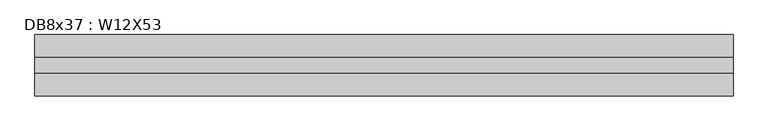
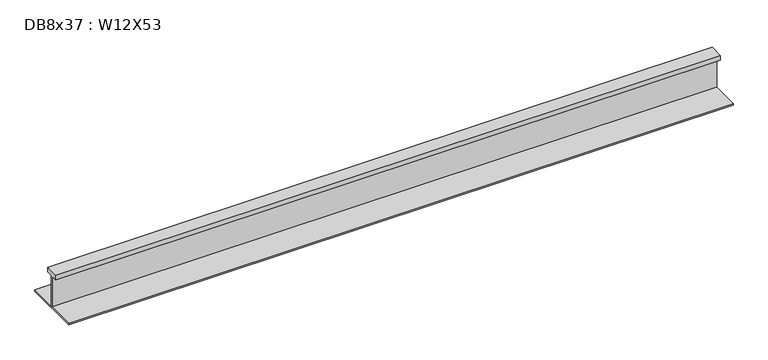
"""IFC4 building model written with IfcOpenShell, lengths in millimetres: beam geometry, DB8x37 : W12X53."""

from ifc_helpers import new_model, si_unit, frame, origin, place, context, project, spatial, polyline, outline, extrude, source, transform, mapped, element, save


def db8x37_w12x53_a618b606(model_context):
    return source(origin(), model_context, "Body", "SweptSolid", [
        extrude(outline(polyline([(38.1, 145.415), (38.1, 120.015), (2.921, 120.015), (2.921, -48.4505), (152.4, -48.4505), (152.4, -58.1025), (-152.4, -58.1025), (-152.4, -48.4505), (-2.921, -48.4505), (-2.921, 120.015), (-38.1, 120.015), (-38.1, 145.415), (38.1, 145.415)])), frame((-1734.5380064, 0.0, 0.0), z_axis=(1.0, 0.0, 0.0), x_axis=(0.0, 1.0, 0.0)), (0.0, 0.0, 1.0), 3466.6542939),
    ])


if __name__ == "__main__":
    model = new_model("IFC4")
    model_context = context("Model", 3, world=origin())
    ifc_project = project(units=[si_unit("LENGTHUNIT", "METRE", prefix="MILLI")], contexts=[model_context])
    site = spatial("IfcSite", under=ifc_project)
    building = spatial("IfcBuilding", under=site)
    placement = place(None, origin())
    db8x37_w12x53_shape = db8x37_w12x53_a618b606(model_context)
    element("IfcBeam", 1, ObjectType="DB8x37 : W12X53", at=placement, inside=building, context=model_context, shape_type="MappedRepresentation", body=[
        mapped(db8x37_w12x53_shape, transform((0.0, 0.0, 0.0), x_axis=(1.0, 0.0, 0.0), y_axis=(0.0, 1.0, 0.0), z_axis=(0.0, 0.0, 1.0))),
    ])
    save(model, "model.ifc")

# Revit data of these elements
# Type "DB8x37 : W12X53"
#   Assembly Code = "B10"
#   W = 53
#   Length [instance default] = 5' - 0"
#   bf = 0' - 10"
#   d = 1' - 0.1"
#   k = 0' - 1 3/8"
#   k2 = 0' - 0.8"
#   tf = 0' - 0.575"
#   tw = 0' - 0.345"
#   A = 0.108333 SF
#   Structural Material [instance default] = Steel ASTM A992
# Element 1 (IfcBeam, "DB8x37 : W12X53")
#   Materials on its faces: "Steel ASTM A992"
# Materials
#   "Steel ASTM A992": class "Metal", colour RGB 199 199 199, transparency 0, Description = "Structural steel 50ksi", Cost = 0
